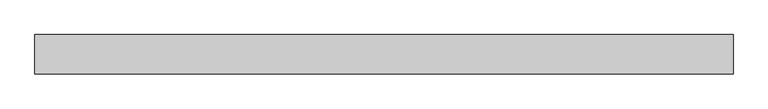
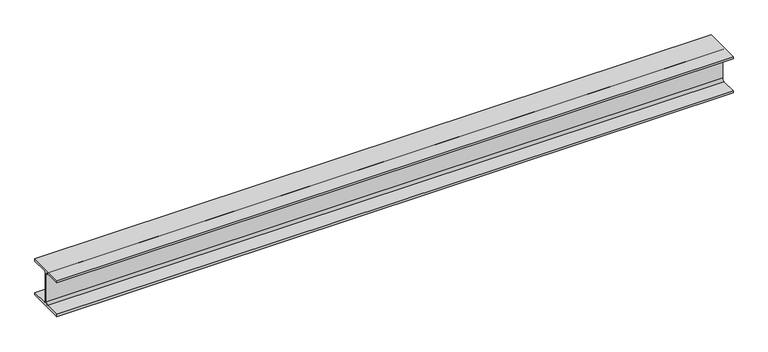
"""IFC4 building model written with IfcOpenShell, lengths in millimetres: beam geometry, 0912_Steel Framing_H-KSD3502 : H_SB_ASB_H-200x200x8x12."""

from ifc_helpers import new_model, si_unit, point, frame, frame_2d, origin, place, context, project, spatial, polyline, circle_curve, trimmed, segment, composite_curve, outline, extrude, source, transform, mapped, element, save


def beam_9e25a490(model_context):
    return source(origin(), model_context, "Body", "SweptSolid", [
        extrude(outline(composite_curve([segment(polyline([(100.0, -88.0), (100.0, -100.0), (-100.0, -100.0), (-100.0, -88.0), (-17.0, -88.0)]), True, "CONTINUOUS"), segment(trimmed(circle_curve(frame_2d((-17.0, -75.0)), 13.0), [point((-17.0, -88.0))], [point((-4.0, -75.0))], True, "CARTESIAN"), True, "CONTINUOUS"), segment(polyline([(-4.0, -75.0), (-4.0, 75.0)]), True, "CONTINUOUS"), segment(trimmed(circle_curve(frame_2d((-17.0, 75.0)), 13.0), [point((-4.0, 75.0))], [point((-17.0, 88.0))], True, "CARTESIAN"), True, "CONTINUOUS"), segment(polyline([(-17.0, 88.0), (-100.0, 88.0), (-100.0, 100.0), (100.0, 100.0), (100.0, 88.0), (17.0, 88.0)]), True, "CONTINUOUS"), segment(trimmed(circle_curve(frame_2d((17.0, 75.0)), 13.0), [point((17.0, 88.0))], [point((4.0, 75.0))], True, "CARTESIAN"), True, "CONTINUOUS"), segment(polyline([(4.0, 75.0), (4.0, -75.0)]), True, "CONTINUOUS"), segment(trimmed(circle_curve(frame_2d((17.0, -75.0)), 13.0), [point((4.0, -75.0))], [point((17.0, -88.0))], True, "CARTESIAN"), True, "CONTINUOUS"), segment(polyline([(17.0, -88.0), (100.0, -88.0)]), True, "CONTINUOUS")], self_intersect=False)), frame((-1734.3504002, 0.0, 0.0), z_axis=(1.0, 0.0, 0.0), x_axis=(0.0, 1.0, 0.0)), (0.0, 0.0, 1.0), 3554.555596),
    ])


if __name__ == "__main__":
    model = new_model("IFC4")
    model_context = context("Model", 3, world=origin())
    ifc_project = project(units=[si_unit("LENGTHUNIT", "METRE", prefix="MILLI")], contexts=[model_context])
    site = spatial("IfcSite", under=ifc_project)
    building = spatial("IfcBuilding", under=site)
    placement = place(None, origin())
    beam_shape = beam_9e25a490(model_context)
    element("IfcBeam", 1, ObjectType="0912_Steel Framing_H-KSD3502 : H_SB_ASB_H-200x200x8x12", at=placement, inside=building, context=model_context, shape_type="MappedRepresentation", body=[
        mapped(beam_shape, transform((0.0, 0.0, 0.0), x_axis=(1.0, 0.0, 0.0), y_axis=(0.0, 1.0, 0.0), z_axis=(0.0, 0.0, 1.0))),
    ])
    save(model, "model.ifc")

# Revit data of these elements
# Type "0912_Steel Framing_H-KSD3502 : H_SB_ASB_H-200x200x8x12"
#   H_WM Code_1 = "S01AA002-00001 | Main Steel Structure Fabrication Work | Shelter/Building | Medium Steel - Standard (90KG/M>Weight≥30KG/M) | Material: (   )"
#   H_WM Code_2 = "S03AA028-00001 | Main Steel Structure Erection Work | Shelter/Building | Medium Steel (90KG/M>Weight≥30KG/M) | Material: (   )"
#   H_WM Code_3 = "S01AA010-00001 | Main Steel Structure Fabrication Work | Shelter/Building | Steel Painting/Coating | for Non-Fireproofed Steel Surface, Surface Preparation, Primer, Second & Final Coat | Material: (   )"
#   H_Q'ty Cal Type Tag = "SB-Q2"
#   Width = 20.0 cm
#   Web Thickness = 0.8 cm
#   Web Fillet = 1.3 cm
#   Warping Constant = 141000.0 cm⁶
#   W = 0
#   Torsional Moment of Inertia = 26.2485 cm⁴
#   Section Area = 63.53 cm²
#   Plastic Modulus weak axis = 244.0 cm³
#   Plastic Modulus strong axis = 525.0 cm³
#   Perimeter = 1.16 m²/m
#   Nominal Weight = 49.90 kgf/m
#   Moment of Inertia weak axis = 1600.00 cm⁴
#   Moment of Inertia strong axis = 4720.00 cm⁴
#   Height = 20.0 cm
#   Flange Thickness = 1.2 cm
#   Elastic Modulus weak axis = 160.0 cm³
#   Elastic Modulus strong axis = 472.0 cm³
#   Centroid Vertical = 10.0 cm
#   Centroid Horizontal = 10.0 cm
#   Ix = 47200000
#   Length [instance default] = 1.5240 m
#   Zx = 525000
#   b = 0.2000 m
#   h = 0.2000 m
#   r = 0.0130 m
#   s = 0.0080 m
#   t = 0.0120 m
#   A = 0.006353 m²
#   Structural Material [instance default] = Steel, 45-345
#   Assembly Code = ""
# Element 1 (IfcBeam, "0912_Steel Framing_H-KSD3502 : H_SB_ASB_H-200x200x8x12")
#   Structural Material = none
# Materials
#   "Steel, 45-345": class "Metal", colour RGB 189 187 185, transparency 0, Description = "Steel 345 MPa", Cost = 0
